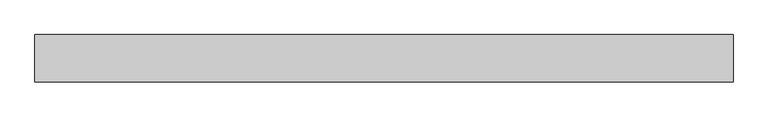
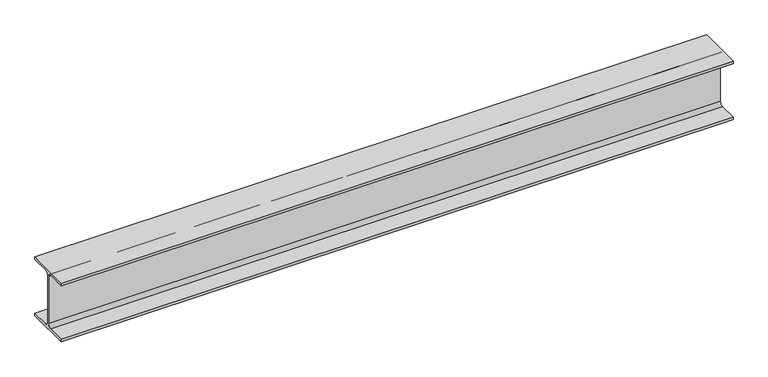
"""IFC4 building model written with IfcOpenShell, lengths in millimetres: beam geometry, 0912_Steel Framing_H-KSD3502 : H_SB_ASB_H-340x250x9x14."""

import ifcopenshell
import ifcopenshell.guid

model = None  # the IFC model being written
_history = None  # IfcOwnerHistory: only IFC2X3 demands one
_inside = {}  # id of a spatial element -> (the spatial element, [elements in it])
_under = {}  # id of a project, library or spatial element -> (it, [spatial elements below it])
_declared = {}  # id of a project -> (the project, [libraries it declares])
_typed = {}  # id of a type object -> (the type object, [elements of that type])
_made_of = {}  # id of a material, layer set ... -> (it, [elements and type objects made of it])


def new_model(schema):
    """Start an empty IFC model of exactly this schema.

    Asked for "IFC4X3", IfcOpenShell would pick the latest addendum, in which some entities
    have other attributes; the version numbers below select the first issue.
    IFC2X3 requires an IfcOwnerHistory on every rooted entity: one is made here for all.
    """
    global model, _history
    if schema == "IFC4X3":
        model = ifcopenshell.file(schema_version=(4, 3, 0, 0))
    else:
        model = ifcopenshell.file(schema=schema)
    _inside.clear()
    _under.clear()
    _declared.clear()
    _typed.clear()
    _made_of.clear()
    _history = None
    if model.schema == "IFC2X3":
        org = make("IfcOrganization", Name="unknown")
        user = make(
            "IfcPersonAndOrganization",
            ThePerson=make("IfcPerson", FamilyName="unknown"),
            TheOrganization=org,
        )
        app = make(
            "IfcApplication",
            ApplicationDeveloper=org,
            Version="unknown",
            ApplicationFullName="unknown",
            ApplicationIdentifier="unknown",
        )
        _history = make(
            "IfcOwnerHistory",
            OwningUser=user,
            OwningApplication=app,
            ChangeAction="ADDED",
            CreationDate=0,
        )
    return model


def make(cls, **values):
    """One entity of the class cls with the attributes given. An attribute that is None is left unset."""
    return model.create_entity(
        cls, **{name: value for name, value in values.items() if value is not None}
    )


def rooted(cls, **values):
    """An entity with a GlobalId (a new one), such as an element, a storey or a relation."""
    return make(cls, GlobalId=ifcopenshell.guid.new(), OwnerHistory=_history, **values)


def si_unit(unit_type, name, prefix=None):
    """IfcSIUnit, for example si_unit("LENGTHUNIT", "METRE", prefix="MILLI")."""
    return make("IfcSIUnit", UnitType=unit_type, Prefix=prefix, Name=name)


def assignment(units):
    """IfcUnitAssignment: the units of a project."""
    return None if units is None else make("IfcUnitAssignment", Units=units)


def point(xyz):
    """IfcCartesianPoint."""
    return None if xyz is None else make("IfcCartesianPoint", Coordinates=xyz)


def direction(xyz):
    """IfcDirection."""
    return None if xyz is None else make("IfcDirection", DirectionRatios=xyz)


def frame(location, z_axis=None, x_axis=None):
    """IfcAxis2Placement3D, a coordinate frame: its origin and axes. An axis left out is left unset."""
    return make(
        "IfcAxis2Placement3D",
        Location=point(location),
        Axis=direction(z_axis),
        RefDirection=direction(x_axis),
    )


def frame_2d(location, x_axis=None):
    """IfcAxis2Placement2D, a coordinate frame in the plane: its origin and x axis."""
    return make(
        "IfcAxis2Placement2D", Location=point(location), RefDirection=direction(x_axis)
    )


def origin():
    """The frame at (0, 0, 0) with its axes left unset."""
    return frame((0.0, 0.0, 0.0))


def place(relative_to, where):
    """IfcLocalPlacement: puts the frame where relative to a parent placement (None: the world)."""
    return make(
        "IfcLocalPlacement", PlacementRelTo=relative_to, RelativePlacement=where
    )


def context(
    kind, dimensions, precision=None, world=None, true_north=None, identifier=None
):
    """IfcGeometricRepresentationContext, for example the 3D "Model" context."""
    return make(
        "IfcGeometricRepresentationContext",
        ContextIdentifier=identifier,
        ContextType=kind,
        CoordinateSpaceDimension=dimensions,
        Precision=precision,
        WorldCoordinateSystem=world,
        TrueNorth=true_north,
    )


def project(units=None, contexts=None):
    """IfcProject with its units and contexts."""
    return rooted(
        "IfcProject",
        Name="project",
        RepresentationContexts=contexts,
        UnitsInContext=assignment(units),
    )


def spatial(cls, under=None, at=None, **own):
    """A site, building, storey or space (cls), placed at a placement, below another one or the project."""
    s = rooted(cls, ObjectPlacement=at, **own)
    if under is not None:
        _under.setdefault(under.id(), (under, []))[1].append(s)
    return s


def polyline(points):
    """IfcPolyline through the points."""
    return make("IfcPolyline", Points=[point(p) for p in points])


def circle_curve(where, radius):
    """IfcCircle in the frame where."""
    return make("IfcCircle", Position=where, Radius=radius)


def trimmed(basis, trim1, trim2, sense, master):
    """IfcTrimmedCurve: the piece of a basis curve between two trims."""
    return make(
        "IfcTrimmedCurve",
        BasisCurve=basis,
        Trim1=trim1,
        Trim2=trim2,
        SenseAgreement=sense,
        MasterRepresentation=master,
    )


def segment(curve, same_sense, transition):
    """IfcCompositeCurveSegment."""
    return make(
        "IfcCompositeCurveSegment",
        Transition=transition,
        SameSense=same_sense,
        ParentCurve=curve,
    )


def composite_curve(segments, self_intersect=None):
    """IfcCompositeCurve: segments joined end to end."""
    return make("IfcCompositeCurve", Segments=segments, SelfIntersect=self_intersect)


def outline(outer, holes=None, kind="AREA"):
    """IfcArbitraryClosedProfileDef: a profile drawn as a closed curve; with holes, ...WithVoids."""
    if holes is None:
        return make("IfcArbitraryClosedProfileDef", ProfileType=kind, OuterCurve=outer)
    return make(
        "IfcArbitraryProfileDefWithVoids",
        ProfileType=kind,
        OuterCurve=outer,
        InnerCurves=holes,
    )


def extrude(swept, where, along, depth):
    """IfcExtrudedAreaSolid: the profile swept, set in the frame where, extruded along a direction by depth."""
    return make(
        "IfcExtrudedAreaSolid",
        SweptArea=swept,
        Position=where,
        ExtrudedDirection=direction(along),
        Depth=depth,
    )


def shape(context_of_items, identifier, shape_type, items):
    """IfcShapeRepresentation: the items that make up one representation, for example the "Body"."""
    return make(
        "IfcShapeRepresentation",
        ContextOfItems=context_of_items,
        RepresentationIdentifier=identifier,
        RepresentationType=shape_type,
        Items=items,
    )


def source(mapping_origin, context_of_items, identifier, shape_type, items):
    """IfcRepresentationMap: a shape defined once, which mapped items show again and again."""
    return make(
        "IfcRepresentationMap",
        MappingOrigin=mapping_origin,
        MappedRepresentation=shape(context_of_items, identifier, shape_type, items),
    )


def transform(
    local_origin,
    x_axis=None,
    y_axis=None,
    z_axis=None,
    scale=None,
    scale2=None,
    scale3=None,
    uniform=True,
):
    """IfcCartesianTransformationOperator3D, or its non-uniform kind. x_axis, y_axis, z_axis: its Axis1, 2, 3."""
    if uniform:
        return make(
            "IfcCartesianTransformationOperator3D",
            Axis1=direction(x_axis),
            Axis2=direction(y_axis),
            LocalOrigin=point(local_origin),
            Scale=scale,
            Axis3=direction(z_axis),
        )
    return make(
        "IfcCartesianTransformationOperator3DnonUniform",
        Axis1=direction(x_axis),
        Axis2=direction(y_axis),
        LocalOrigin=point(local_origin),
        Scale=scale,
        Axis3=direction(z_axis),
        Scale2=scale2,
        Scale3=scale3,
    )


def mapped(mapping_source, mapping_target):
    """IfcMappedItem: shows the shape of a source again, moved by a transform."""
    return make(
        "IfcMappedItem", MappingSource=mapping_source, MappingTarget=mapping_target
    )


def made_of(thing, what):
    """Note that an element or type object is made of a material, layer set ...; save() writes the relation."""
    if what is not None:
        _made_of.setdefault(what.id(), (what, []))[1].append(thing)
    return thing


def element(
    cls,
    number,
    at=None,
    inside=None,
    cuts=None,
    type_object=None,
    material=None,
    context=None,
    identifier="Body",
    shape_type=None,
    held_by="IfcProductDefinitionShape",
    body=None,
    shapes=None,
    **own,
):
    """One element of the class cls, such as IfcWall. Its Tag is "e" and its number.

    at: its placement. inside: the storey or other place that contains it. cuts: it is an
    opening in that element (IfcRelVoidsElement). A single representation is given by context,
    identifier, shape_type and body (its items); several are given by shapes. held_by: the class
    of the entity that holds the representations. save() writes the other relations.
    """
    e = rooted(cls, Tag="e%d" % number, ObjectPlacement=at, **own)
    if body is not None:
        shapes = [shape(context, identifier, shape_type, body)]
    if shapes is not None:
        e.Representation = make(held_by, Representations=shapes)
    if inside is not None:
        _inside.setdefault(inside.id(), (inside, []))[1].append(e)
    if cuts is not None:
        rooted(
            "IfcRelVoidsElement", RelatingBuildingElement=cuts, RelatedOpeningElement=e
        )
    if type_object is not None:
        _typed.setdefault(type_object.id(), (type_object, []))[1].append(e)
    return made_of(e, material)


def aggregate(whole, parts):
    """IfcRelAggregates: a whole, such as a stair, and the parts it consists of."""
    return rooted("IfcRelAggregates", RelatingObject=whole, RelatedObjects=parts)


def save(model, path):
    """Write the relations noted so far, then the file.

    IfcRelAggregates (storeys below a building ...), IfcRelContainedInSpatialStructure (elements
    in a storey), IfcRelDefinesByType, IfcRelAssociatesMaterial and IfcRelDeclares: one each for
    every whole, place, type object, material and project.
    """
    for whole, parts in _under.values():
        aggregate(whole, parts)
    for where, things in _inside.values():
        rooted(
            "IfcRelContainedInSpatialStructure",
            RelatedElements=things,
            RelatingStructure=where,
        )
    for kind, things in _typed.values():
        rooted("IfcRelDefinesByType", RelatedObjects=things, RelatingType=kind)
    for what, things in _made_of.values():
        rooted("IfcRelAssociatesMaterial", RelatedObjects=things, RelatingMaterial=what)
    for by, libraries in _declared.values():
        rooted("IfcRelDeclares", RelatingContext=by, RelatedDefinitions=libraries)
    model.write(path)


def beam_4526978a(model_context):
    return source(origin(), model_context, "Body", "SweptSolid", [
        extrude(outline(composite_curve([segment(polyline([(125.0, -156.0), (125.0, -170.0), (-125.0, -170.0), (-125.0, -156.0), (-24.5, -156.0)]), True, "CONTINUOUS"), segment(trimmed(circle_curve(frame_2d((-24.5, -136.0)), 20.0), [point((-24.5, -156.0))], [point((-4.5, -136.0))], True, "CARTESIAN"), True, "CONTINUOUS"), segment(polyline([(-4.5, -136.0), (-4.5, 136.0)]), True, "CONTINUOUS"), segment(trimmed(circle_curve(frame_2d((-24.5, 136.0)), 20.0), [point((-4.5, 136.0))], [point((-24.5, 156.0))], True, "CARTESIAN"), True, "CONTINUOUS"), segment(polyline([(-24.5, 156.0), (-125.0, 156.0), (-125.0, 170.0), (125.0, 170.0), (125.0, 156.0), (24.5, 156.0)]), True, "CONTINUOUS"), segment(trimmed(circle_curve(frame_2d((24.5, 136.0)), 20.0), [point((24.5, 156.0))], [point((4.5, 136.0))], True, "CARTESIAN"), True, "CONTINUOUS"), segment(polyline([(4.5, 136.0), (4.5, -136.0)]), True, "CONTINUOUS"), segment(trimmed(circle_curve(frame_2d((24.5, -136.0)), 20.0), [point((4.5, -136.0))], [point((24.5, -156.0))], True, "CARTESIAN"), True, "CONTINUOUS"), segment(polyline([(24.5, -156.0), (125.0, -156.0)]), True, "CONTINUOUS")], self_intersect=False)), frame((-1837.3, 0.0, 0.0), z_axis=(1.0, 0.0, 0.0), x_axis=(0.0, 1.0, 0.0)), (0.0, 0.0, 1.0), 3674.6),
    ])


if __name__ == "__main__":
    model = new_model("IFC4")
    model_context = context("Model", 3, world=origin())
    ifc_project = project(units=[si_unit("LENGTHUNIT", "METRE", prefix="MILLI")], contexts=[model_context])
    site = spatial("IfcSite", under=ifc_project)
    building = spatial("IfcBuilding", under=site)
    placement = place(None, origin())
    beam_shape = beam_4526978a(model_context)
    element("IfcBeam", 1, ObjectType="0912_Steel Framing_H-KSD3502 : H_SB_ASB_H-340x250x9x14", at=placement, inside=building, context=model_context, shape_type="MappedRepresentation", body=[
        mapped(beam_shape, transform((0.0, 0.0, 0.0), x_axis=(1.0, 0.0, 0.0), y_axis=(0.0, 1.0, 0.0), z_axis=(0.0, 0.0, 1.0))),
    ])
    save(model, "model.ifc")

# Revit data of these elements
# Type "0912_Steel Framing_H-KSD3502 : H_SB_ASB_H-340x250x9x14"
#   H_WM Code_1 = "S01AA002-00001 | Main Steel Structure Fabrication Work | Shelter/Building | Medium Steel - Standard (90KG/M>Weight≥30KG/M) | Material: (   )"
#   H_WM Code_2 = "S03AA028-00001 | Main Steel Structure Erection Work | Shelter/Building | Medium Steel (90KG/M>Weight≥30KG/M) | Material: (   )"
#   H_WM Code_3 = "S01AA010-00001 | Main Steel Structure Fabrication Work | Shelter/Building | Steel Painting/Coating | for Non-Fireproofed Steel Surface, Surface Preparation, Primer, Second & Final Coat | Material: (   )"
#   H_Q'ty Cal Type Tag = "SB-Q2"
#   Width = 25.0 cm
#   Web Thickness = 0.9 cm
#   Web Fillet = 2.0 cm
#   Warping Constant = 969000.0 cm⁶
#   W = 0
#   Torsional Moment of Inertia = 53.6551 cm⁴
#   Section Area = 101.5 cm²
#   Plastic Modulus weak axis = 447.0 cm³
#   Plastic Modulus strong axis = 1410.0 cm³
#   Perimeter = 1.63 m²/m
#   Nominal Weight = 79.70 kgf/m
#   Moment of Inertia weak axis = 3650.00 cm⁴
#   Moment of Inertia strong axis = 21700.00 cm⁴
#   Height = 34.0 cm
#   Flange Thickness = 1.4 cm
#   Elastic Modulus weak axis = 292.0 cm³
#   Elastic Modulus strong axis = 1280.0 cm³
#   Centroid Vertical = 17.0 cm
#   Centroid Horizontal = 12.5 cm
#   Ix = 217000000
#   Length [instance default] = 1.5240 m
#   Zx = 1410000
#   b = 0.2500 m
#   h = 0.3400 m
#   r = 0.0200 m
#   s = 0.0090 m
#   t = 0.0140 m
#   A = 0.01015 m²
#   Structural Material [instance default] = Steel, 45-345
#   Assembly Code = ""
# Element 1 (IfcBeam, "0912_Steel Framing_H-KSD3502 : H_SB_ASB_H-340x250x9x14")
#   Structural Material = none
# Materials
#   "Steel, 45-345": class "Metal", colour RGB 189 187 185, transparency 0, Description = "Steel 345 MPa", Cost = 0
